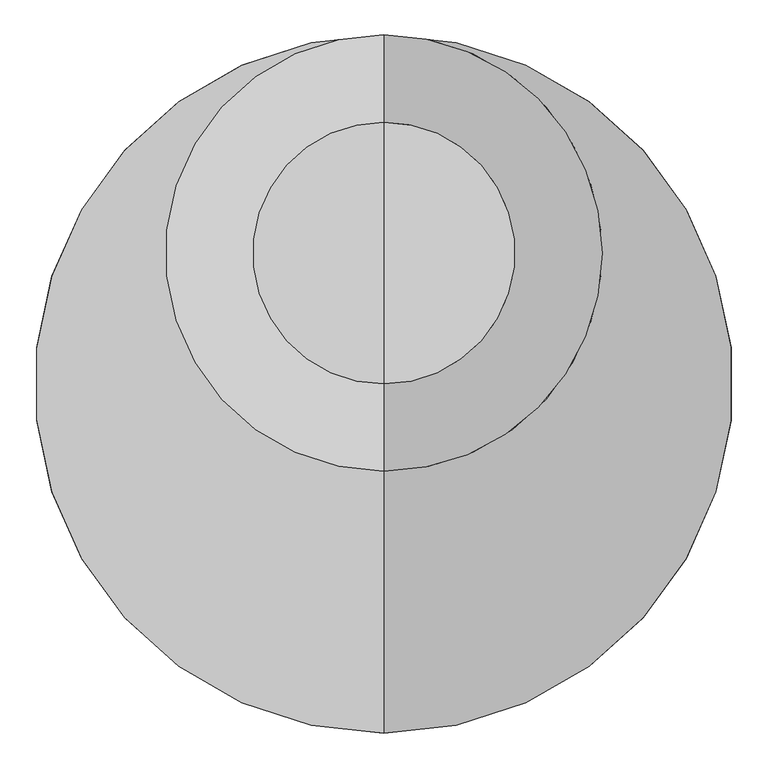
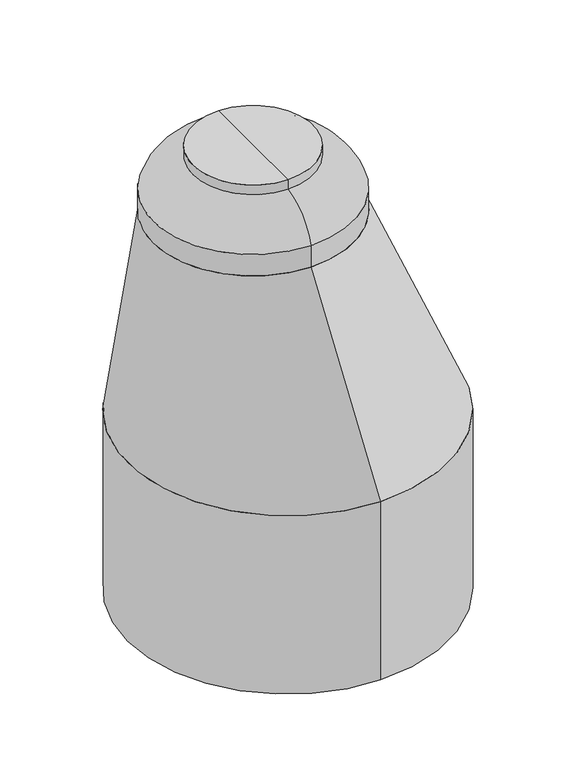
"""IFC4 building model written with IfcOpenShell, lengths in millimetres: proxy geometry, Sewer Manhole - EX_CB : Sewer Manhole - EX_CB."""

from ifc_helpers import new_model, si_unit, point, frame, origin, place, context, project, spatial, circle_curve, ellipse_curve, trimmed, source, transform, mapped, element, save
from ifc_brep_helpers import plane_surface, cylinder_surface, revolved_surface, spline_surface, advanced_brep


def generic_models_880986fa(model_context):
    return source(origin(), model_context, "Body", "AdvancedBrep", [
        advanced_brep(
        [(0.0, 812.8, 1840.7270774), (0.0, -203.2, 1840.7270774), (0.0, 812.8, 955.04), (0.0, -812.8, 955.04)],
        [
            (0, 1, circle_curve(frame((0.0, 304.8, 1840.7270774), z_axis=(0.0, 0.0, 1.0), x_axis=(0.0, 1.0, 0.0)), 508.0)),
            (1, 0, circle_curve(frame((0.0, 304.8, 1840.7270774), z_axis=(0.0, 0.0, 1.0), x_axis=(0.0, 1.0, 0.0)), 508.0)),
            (2, 3, circle_curve(frame((0.0, 0.0, 955.04), z_axis=(0.0, 0.0, -1.0), x_axis=(0.0, 1.0, 0.0)), 812.8)),
            (3, 2, circle_curve(frame((0.0, 0.0, 955.04), z_axis=(0.0, 0.0, -1.0), x_axis=(0.0, 1.0, 0.0)), 812.8)),
            (3, 1),
            (0, 2),
        ],
        [
            plane_surface(frame((0.0, 304.8, 1840.7270774), z_axis=(0.0, 0.0, 1.0), x_axis=(1.0, 0.0, 0.0))),
            plane_surface(frame((0.0, 0.0, 955.04), z_axis=(0.0, 0.0, -1.0), x_axis=(1.0, 0.0, 0.0))),
            spline_surface(2, 1, [[(0.0, 812.8, 955.04), (0.0, 812.8, 1840.7270774)], [(-812.8, 812.8, 955.04), (-507.99999999999994, 812.8, 1840.7270774)], [(-812.8, 0.0, 955.04), (-507.99999999999994, 304.8, 1840.7270774)], [(-812.8, -812.8, 955.04), (-507.99999999999994, -203.19999999999993, 1840.7270774)], [(0.0, -812.8, 955.04), (0.0, -203.2, 1840.7270774)]], [3, 2, 3], [2, 2], [0.0, 1.0, 2.0], [0.0, 1.0], weights=[[1.0, 1.0], [0.7071067811865476, 0.7071067811865476], [1.0, 1.0], [0.7071067811865476, 0.7071067811865476], [1.0, 1.0]]),
            spline_surface(2, 1, [[(0.0, -812.8, 955.04), (0.0, -203.2, 1840.7270774)], [(812.8, -812.8, 955.04), (508.0, -203.2, 1840.7270774)], [(812.8, 0.0, 955.04), (508.0, 304.8, 1840.7270774)], [(812.8, 812.8, 955.04), (508.0, 812.8, 1840.7270774)], [(0.0, 812.8, 955.04), (0.0, 812.8, 1840.7270774)]], [3, 2, 3], [2, 2], [0.0, 1.0, 2.0], [0.0, 1.0], weights=[[1.0, 1.0], [0.7071067811865476, 0.7071067811865476], [1.0, 1.0], [0.7071067811865476, 0.7071067811865476], [1.0, 1.0]]),
        ],
        [
            (0, [[1, 2]]),
            (1, [[3, 4]]),
            (2, [[-4, 5, -1, 6]]),
            (3, [[-3, -6, -2, -5]]),
        ],
    ),
        advanced_brep(
        [(0.0, -203.2, 1840.7270774), (0.0, 812.8, 1840.7270774), (0.0, 304.8, 1840.7270774), (0.0, -203.2, 1955.8), (0.0, 812.8, 1955.8), (0.0, 0.0, 2133.6), (0.0, 609.6, 2133.6), (0.0, 0.0, 2184.4), (0.0, 609.6, 2184.4), (0.0, 304.8, 2184.4)],
        [
            (0, 1, circle_curve(frame((0.0, 304.8, 1840.7270774), z_axis=(0.0, 0.0, -1.0), x_axis=(0.0, 1.0, 0.0)), 508.0)),
            (1, 2),
            (2, 0),
            (1, 0, circle_curve(frame((0.0, 304.8, 1840.7270774), z_axis=(0.0, 0.0, -1.0), x_axis=(0.0, 1.0, 0.0)), 508.0)),
            (3, 4, circle_curve(frame((0.0, 304.8, 1955.8), z_axis=(0.0, 0.0, -1.0), x_axis=(0.0, 1.0, 0.0)), 508.0)),
            (4, 1),
            (0, 3),
            (4, 3, circle_curve(frame((0.0, 304.8, 1955.8), z_axis=(0.0, 0.0, -1.0), x_axis=(0.0, 1.0, 0.0)), 508.0)),
            (5, 6, circle_curve(frame((0.0, 304.8, 2133.6), z_axis=(0.0, 0.0, -1.0), x_axis=(0.0, 1.0, 0.0)), 304.8)),
            (6, 4, circle_curve(frame((0.0, 564.4539436, 1876.9902213), z_axis=(-1.0, 0.0, 0.0), x_axis=(0.0, -1.0, 0.0)), 260.550849)),
            (3, 5, circle_curve(frame((0.0, 45.1460564, 1876.9902213), z_axis=(-1.0, 0.0, 0.0), x_axis=(0.0, 1.0, 0.0)), 260.550849)),
            (6, 5, circle_curve(frame((0.0, 304.8, 2133.6), z_axis=(0.0, 0.0, -1.0), x_axis=(0.0, 1.0, 0.0)), 304.8)),
            (7, 8, circle_curve(frame((0.0, 304.8, 2184.4), z_axis=(0.0, 0.0, -1.0), x_axis=(0.0, 1.0, 0.0)), 304.8)),
            (8, 6),
            (5, 7),
            (8, 7, circle_curve(frame((0.0, 304.8, 2184.4), z_axis=(0.0, 0.0, -1.0), x_axis=(0.0, 1.0, 0.0)), 304.8)),
            (9, 8),
            (7, 9),
        ],
        [
            plane_surface(frame((0.0, 304.8, 1840.7270774), z_axis=(0.0, 0.0, -1.0), x_axis=(0.0, 1.0, 0.0))),
            cylinder_surface(frame((0.0, 304.8, 1905.0), z_axis=(0.0, 0.0, 1.0), x_axis=(0.0, 1.0, 0.0)), 508.0),
            revolved_surface(trimmed(ellipse_curve(frame((0.0, 564.4539436, 1876.9902213), z_axis=(1.0, 0.0, 0.0), x_axis=(0.0, -1.0, 0.0)), 260.550849, 260.550849), [point((0.0, 812.8, 1955.8))], [point((0.0, 609.6, 2133.6))], True, "CARTESIAN"), (0.0, 304.8, 1905.0), (0.0, 0.0, 1.0)),
            cylinder_surface(frame((0.0, 304.8, 1905.0), z_axis=(0.0, 0.0, 1.0), x_axis=(0.0, 1.0, 0.0)), 304.8),
            plane_surface(frame((0.0, 304.8, 2184.4), z_axis=(0.0, 0.0, 1.0), x_axis=(0.0, 1.0, 0.0))),
        ],
        [
            (0, [[1, 2, 3]]),
            (0, [[4, -3, -2]]),
            (1, [[5, 6, -1, 7]]),
            (1, [[8, -7, -4, -6]]),
            (2, [[9, 10, -5, 11]]),
            (2, [[12, -11, -8, -10]]),
            (3, [[13, 14, -9, 15]]),
            (3, [[16, -15, -12, -14]]),
            (4, [[17, -13, 18]]),
            (4, [[-18, -16, -17]]),
        ],
    ),
        advanced_brep(
        [(0.0, -812.8, 955.04), (0.0, 812.8, 955.04), (0.0, 812.8, 0.0), (0.0, -812.8, 0.0), (0.0, 0.0, 0.0), (0.0, 0.0, 955.04)],
        [
            (0, 1, circle_curve(frame((0.0, 0.0, 955.04), z_axis=(0.0, 0.0, -1.0), x_axis=(0.0, 1.0, 0.0)), 812.8)),
            (1, 2),
            (2, 3, circle_curve(frame((0.0, 0.0, 0.0), z_axis=(0.0, 0.0, 1.0), x_axis=(0.0, 1.0, 0.0)), 812.8)),
            (3, 0),
            (1, 0, circle_curve(frame((0.0, 0.0, 955.04), z_axis=(0.0, 0.0, -1.0), x_axis=(0.0, 1.0, 0.0)), 812.8)),
            (3, 2, circle_curve(frame((0.0, 0.0, 0.0), z_axis=(0.0, 0.0, 1.0), x_axis=(0.0, 1.0, 0.0)), 812.8)),
            (2, 4),
            (4, 3),
            (5, 1),
            (0, 5),
        ],
        [
            cylinder_surface(frame((0.0, 0.0, 457.2), z_axis=(0.0, 0.0, 1.0), x_axis=(0.0, 1.0, 0.0)), 812.8),
            plane_surface(frame((0.0, 0.0, 0.0), z_axis=(0.0, 0.0, -1.0), x_axis=(0.0, 1.0, 0.0))),
            plane_surface(frame((0.0, 0.0, 955.04), z_axis=(0.0, 0.0, 1.0), x_axis=(0.0, 1.0, 0.0))),
        ],
        [
            (0, [[1, 2, 3, 4]]),
            (0, [[5, -4, 6, -2]]),
            (1, [[-3, 7, 8]]),
            (1, [[-6, -8, -7]]),
            (2, [[9, -1, 10]]),
            (2, [[-10, -5, -9]]),
        ],
    ),
    ])


if __name__ == "__main__":
    model = new_model("IFC4")
    model_context = context("Model", 3, world=origin())
    ifc_project = project(units=[si_unit("LENGTHUNIT", "METRE", prefix="MILLI")], contexts=[model_context])
    site = spatial("IfcSite", under=ifc_project)
    building = spatial("IfcBuilding", under=site)
    placement = place(None, origin())
    generic_models_shape = generic_models_880986fa(model_context)
    element("IfcBuildingElementProxy", 1, Name="Sewer Manhole - EX_CB : Sewer Manhole - EX_CB", ObjectType="Sewer Manhole - EX_CB : Sewer Manhole - EX_CB", at=placement, inside=building, context=model_context, shape_type="MappedRepresentation", body=[
        mapped(generic_models_shape, transform((0.0, 0.0, 0.0), x_axis=(1.0, 0.0, 0.0), y_axis=(0.0, 1.0, 0.0), z_axis=(0.0, 0.0, 1.0))),
    ])
    save(model, "model.ifc")
